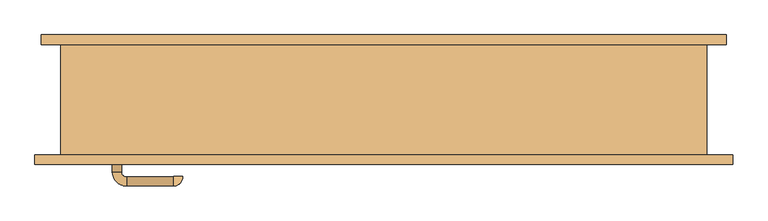
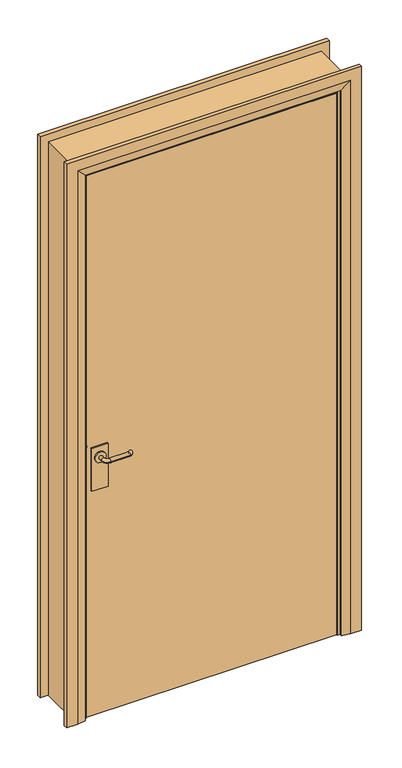
"""IFC4 building model written with IfcOpenShell, lengths in millimetres: door geometry, Porta Simples de Abrir : 90x210cm - Marco de Madeira."""

from ifc_helpers import new_model, si_unit, point, frame, frame_2d, origin, place, context, project, spatial, polyline, circle_curve, ellipse_curve, trimmed, segment, composite_curve, outline, extrude, faceted_brep, source, transform, mapped, element, save
from ifc_brep_helpers import plane_surface, cylinder_surface, revolved_surface, advanced_brep


def door_5ffc7892(model_context):
    return source(origin(), model_context, "Body", "SolidModel", [
        extrude(outline(composite_curve([segment(trimmed(circle_curve(frame_2d((1050.0, -413.0)), 20.0), [point((1050.0, -433.0))], [point((1050.0, -393.0))], False, "CARTESIAN"), True, "CONTINUOUS"), segment(trimmed(circle_curve(frame_2d((1050.0, -413.0)), 20.0), [point((1050.0, -393.0))], [point((1050.0, -433.0))], False, "CARTESIAN"), True, "CONTINUOUS")], self_intersect=False)), frame((0.0, -44.6, 0.0), z_axis=(0.0, 1.0, 0.0), x_axis=(0.0, 0.0, 1.0)), (0.0, 0.0, 1.0), 4.5929895),
        advanced_brep(
        [(-406.0, -40.0070105, 1050.0), (-420.0, -40.0070105, 1050.0), (-406.0, -24.6, 1050.0), (-420.0, -24.6, 1050.0), (-398.0, -2.6, 1050.0), (-398.0, -16.6, 1050.0), (-326.0, -16.6, 1050.0), (-326.0, -2.6, 1050.0), (-325.0, -17.6, 1050.0), (-311.0, -17.6, 1050.0)],
        [
            (0, 1, circle_curve(frame((-413.0, -40.0070105, 1050.0), z_axis=(0.0, -1.0, 0.0), x_axis=(-1.0, 0.0, 0.0)), 7.0)),
            (1, 0, circle_curve(frame((-413.0, -40.0070105, 1050.0), z_axis=(0.0, -1.0, 0.0), x_axis=(-1.0, 0.0, 0.0)), 7.0)),
            (0, 2),
            (2, 3, circle_curve(frame((-413.0, -24.6, 1050.0), z_axis=(0.0, -1.0, 0.0), x_axis=(-1.0, 0.0, 0.0)), 7.0)),
            (3, 1),
            (3, 2, circle_curve(frame((-413.0, -24.6, 1050.0), z_axis=(0.0, -1.0, 0.0), x_axis=(-1.0, 0.0, 0.0)), 7.0)),
            (4, 3, circle_curve(frame((-398.0, -24.6, 1050.0), z_axis=(0.0, 0.0, 1.0), x_axis=(-1.0, 0.0, 0.0)), 22.0)),
            (2, 5, circle_curve(frame((-398.0, -24.6, 1050.0), z_axis=(0.0, 0.0, -1.0), x_axis=(-1.0, 0.0, 0.0)), 8.0)),
            (5, 4, circle_curve(frame((-398.0, -9.6, 1050.0), z_axis=(-1.0, 0.0, 0.0), x_axis=(0.0, 1.0, 0.0)), 7.0)),
            (4, 5, circle_curve(frame((-398.0, -9.6, 1050.0), z_axis=(-1.0, 0.0, 0.0), x_axis=(0.0, 1.0, 0.0)), 7.0)),
            (5, 6),
            (6, 7, circle_curve(frame((-326.0, -9.6, 1050.0), z_axis=(-1.0, 0.0, 0.0), x_axis=(0.0, 1.0, 0.0)), 7.0)),
            (7, 4),
            (7, 6, circle_curve(frame((-326.0, -9.6, 1050.0), z_axis=(-1.0, 0.0, 0.0), x_axis=(0.0, 1.0, 0.0)), 7.0)),
            (8, 9, circle_curve(frame((-318.0, -17.6, 1050.0), z_axis=(0.0, -1.0, 0.0), x_axis=(1.0, 0.0, 0.0)), 7.0)),
            (9, 8, circle_curve(frame((-318.0, -17.6, 1050.0), z_axis=(0.0, -1.0, 0.0), x_axis=(1.0, 0.0, 0.0)), 7.0)),
            (9, 7, circle_curve(frame((-326.0, -17.6, 1050.0), z_axis=(0.0, 0.0, 1.0), x_axis=(0.0, 1.0, 0.0)), 15.0)),
            (6, 8, circle_curve(frame((-326.0, -17.6, 1050.0), z_axis=(0.0, 0.0, -1.0), x_axis=(0.0, 1.0, 0.0)), 1.0)),
        ],
        [
            plane_surface(frame((-413.0, -40.0070105, 1050.0), z_axis=(0.0, -1.0, 0.0), x_axis=(0.0, 0.0, 1.0))),
            cylinder_surface(frame((-413.0, -40.0070105, 1050.0), z_axis=(0.0, -1.0, 0.0), x_axis=(-1.0, 0.0, 0.0)), 7.0),
            revolved_surface(trimmed(ellipse_curve(frame((-413.0, -24.6, 1050.0), z_axis=(0.0, -1.0, 0.0), x_axis=(-1.0, 0.0, 0.0)), 7.0, 7.0), [point((-406.0, -24.6, 1050.0))], [point((-420.0, -24.6, 1050.0))], True, "CARTESIAN"), (-398.0, -24.6, 1050.0), (0.0, 0.0, -1.0)),
            revolved_surface(trimmed(ellipse_curve(frame((-413.0, -24.6, 1050.0), z_axis=(0.0, -1.0, 0.0), x_axis=(-1.0, 0.0, 0.0)), 7.0, 7.0), [point((-420.0, -24.6, 1050.0))], [point((-406.0, -24.6, 1050.0))], True, "CARTESIAN"), (-398.0, -24.6, 1050.0), (0.0, 0.0, -1.0)),
            cylinder_surface(frame((-398.0, -9.6, 1050.0), z_axis=(-1.0, 0.0, 0.0), x_axis=(0.0, 1.0, 0.0)), 7.0),
            plane_surface(frame((-318.0, -17.6, 1050.0), z_axis=(0.0, -1.0, 0.0), x_axis=(0.0, 0.0, 1.0))),
            revolved_surface(trimmed(ellipse_curve(frame((-326.0, -9.6, 1050.0), z_axis=(-1.0, 0.0, 0.0), x_axis=(0.0, 1.0, 0.0)), 7.0, 7.0), [point((-326.0, -16.6, 1050.0))], [point((-326.0, -2.6, 1050.0))], True, "CARTESIAN"), (-326.0, -17.6, 1050.0), (0.0, 0.0, -1.0)),
            revolved_surface(trimmed(ellipse_curve(frame((-326.0, -9.6, 1050.0), z_axis=(-1.0, 0.0, 0.0), x_axis=(0.0, 1.0, 0.0)), 7.0, 7.0), [point((-326.0, -2.6, 1050.0))], [point((-326.0, -16.6, 1050.0))], True, "CARTESIAN"), (-326.0, -17.6, 1050.0), (0.0, 0.0, -1.0)),
        ],
        [
            (0, [[1, 2]]),
            (1, [[-1, 3, 4, 5]]),
            (1, [[-2, -5, 6, -3]]),
            (2, [[7, -4, 8, 9]]),
            (3, [[-8, -6, -7, 10]]),
            (4, [[-9, 11, 12, 13]]),
            (4, [[-10, -13, 14, -11]]),
            (5, [[15, 16]]),
            (6, [[17, -12, 18, -16]]),
            (7, [[-18, -14, -17, -15]]),
        ],
    ),
        extrude(outline(polyline([(-383.0, -50.6), (-443.0, -50.6), (-443.0, -44.6), (-383.0, -44.6), (-383.0, -50.6)])), frame((0.0, 0.0, 925.0), z_axis=(0.0, 0.0, 1.0), x_axis=(1.0, 0.0, 0.0)), (0.0, 0.0, 1.0), 165.0),
        extrude(outline(composite_curve([segment(trimmed(circle_curve(frame_2d((1050.0, -413.0)), 20.0), [point((1050.0, -433.0))], [point((1050.0, -393.0))], False, "CARTESIAN"), True, "CONTINUOUS"), segment(trimmed(circle_curve(frame_2d((1050.0, -413.0)), 20.0), [point((1050.0, -393.0))], [point((1050.0, -433.0))], False, "CARTESIAN"), True, "CONTINUOUS")], self_intersect=False)), frame((0.0, -96.1929895, 0.0), z_axis=(0.0, 1.0, 0.0), x_axis=(0.0, 0.0, 1.0)), (0.0, 0.0, 1.0), 4.5929895),
        advanced_brep(
        [(-406.0, -96.1929895, 1050.0), (-420.0, -96.1929895, 1050.0), (-420.0, -111.6, 1050.0), (-406.0, -111.6, 1050.0), (-398.0, -133.6, 1050.0), (-398.0, -119.6, 1050.0), (-326.0, -133.6, 1050.0), (-326.0, -119.6, 1050.0), (-325.0, -118.6, 1050.0), (-311.0, -118.6, 1050.0)],
        [
            (0, 1, circle_curve(frame((-413.0, -96.1929895, 1050.0), z_axis=(0.0, 1.0, 0.0), x_axis=(-1.0, 0.0, 0.0)), 7.0)),
            (1, 0, circle_curve(frame((-413.0, -96.1929895, 1050.0), z_axis=(0.0, 1.0, 0.0), x_axis=(-1.0, 0.0, 0.0)), 7.0)),
            (1, 2),
            (2, 3, circle_curve(frame((-413.0, -111.6, 1050.0), z_axis=(0.0, 1.0, 0.0), x_axis=(-1.0, 0.0, 0.0)), 7.0)),
            (3, 0),
            (3, 2, circle_curve(frame((-413.0, -111.6, 1050.0), z_axis=(0.0, 1.0, 0.0), x_axis=(-1.0, 0.0, 0.0)), 7.0)),
            (4, 5, circle_curve(frame((-398.0, -126.6, 1050.0), z_axis=(-1.0, 0.0, 0.0), x_axis=(0.0, -1.0, 0.0)), 7.0)),
            (5, 3, circle_curve(frame((-398.0, -111.6, 1050.0), z_axis=(0.0, 0.0, -1.0), x_axis=(-1.0, 0.0, 0.0)), 8.0)),
            (2, 4, circle_curve(frame((-398.0, -111.6, 1050.0), z_axis=(0.0, 0.0, 1.0), x_axis=(-1.0, 0.0, 0.0)), 22.0)),
            (5, 4, circle_curve(frame((-398.0, -126.6, 1050.0), z_axis=(-1.0, 0.0, 0.0), x_axis=(0.0, -1.0, 0.0)), 7.0)),
            (4, 6),
            (6, 7, circle_curve(frame((-326.0, -126.6, 1050.0), z_axis=(-1.0, 0.0, 0.0), x_axis=(0.0, -1.0, 0.0)), 7.0)),
            (7, 5),
            (7, 6, circle_curve(frame((-326.0, -126.6, 1050.0), z_axis=(-1.0, 0.0, 0.0), x_axis=(0.0, -1.0, 0.0)), 7.0)),
            (8, 9, circle_curve(frame((-318.0, -118.6, 1050.0), z_axis=(0.0, 1.0, 0.0), x_axis=(1.0, 0.0, 0.0)), 7.0)),
            (9, 8, circle_curve(frame((-318.0, -118.6, 1050.0), z_axis=(0.0, 1.0, 0.0), x_axis=(1.0, 0.0, 0.0)), 7.0)),
            (8, 7, circle_curve(frame((-326.0, -118.6, 1050.0), z_axis=(0.0, 0.0, -1.0), x_axis=(0.0, -1.0, 0.0)), 1.0)),
            (6, 9, circle_curve(frame((-326.0, -118.6, 1050.0), z_axis=(0.0, 0.0, 1.0), x_axis=(0.0, -1.0, 0.0)), 15.0)),
        ],
        [
            plane_surface(frame((-413.0, -96.1929895, 1050.0), z_axis=(0.0, 1.0, 0.0), x_axis=(0.0, 0.0, 1.0))),
            cylinder_surface(frame((-413.0, -96.1929895, 1050.0), z_axis=(0.0, 1.0, 0.0), x_axis=(-1.0, 0.0, 0.0)), 7.0),
            revolved_surface(trimmed(ellipse_curve(frame((-413.0, -111.6, 1050.0), z_axis=(0.0, -1.0, 0.0), x_axis=(-1.0, 0.0, 0.0)), 7.0, 7.0), [point((-406.0, -111.6, 1050.0))], [point((-420.0, -111.6, 1050.0))], True, "CARTESIAN"), (-398.0, -111.6, 1050.0), (0.0, 0.0, -1.0)),
            revolved_surface(trimmed(ellipse_curve(frame((-413.0, -111.6, 1050.0), z_axis=(0.0, -1.0, 0.0), x_axis=(-1.0, 0.0, 0.0)), 7.0, 7.0), [point((-420.0, -111.6, 1050.0))], [point((-406.0, -111.6, 1050.0))], True, "CARTESIAN"), (-398.0, -111.6, 1050.0), (0.0, 0.0, -1.0)),
            cylinder_surface(frame((-398.0, -126.6, 1050.0), z_axis=(-1.0, 0.0, 0.0), x_axis=(0.0, -1.0, 0.0)), 7.0),
            plane_surface(frame((-318.0, -118.6, 1050.0), z_axis=(0.0, 1.0, 0.0), x_axis=(0.0, 0.0, 1.0))),
            revolved_surface(trimmed(ellipse_curve(frame((-326.0, -126.6, 1050.0), z_axis=(1.0, 0.0, 0.0), x_axis=(0.0, -1.0, 0.0)), 7.0, 7.0), [point((-326.0, -119.6, 1050.0))], [point((-326.0, -133.6, 1050.0))], True, "CARTESIAN"), (-326.0, -118.6, 1050.0), (0.0, 0.0, -1.0)),
            revolved_surface(trimmed(ellipse_curve(frame((-326.0, -126.6, 1050.0), z_axis=(1.0, 0.0, 0.0), x_axis=(0.0, -1.0, 0.0)), 7.0, 7.0), [point((-326.0, -133.6, 1050.0))], [point((-326.0, -119.6, 1050.0))], True, "CARTESIAN"), (-326.0, -118.6, 1050.0), (0.0, 0.0, -1.0)),
        ],
        [
            (0, [[1, 2]]),
            (1, [[3, 4, 5, -2]]),
            (1, [[-5, 6, -3, -1]]),
            (2, [[7, 8, -4, 9]]),
            (3, [[10, -9, -6, -8]]),
            (4, [[11, 12, 13, -7]]),
            (4, [[-13, 14, -11, -10]]),
            (5, [[15, 16]]),
            (6, [[-15, 17, -12, 18]]),
            (7, [[-16, -18, -14, -17]]),
        ],
    ),
        extrude(outline(polyline([(-383.0, -85.6), (-383.0, -91.6), (-443.0, -91.6), (-443.0, -85.6), (-383.0, -85.6)])), frame((0.0, 0.0, 925.0), z_axis=(0.0, 0.0, 1.0), x_axis=(1.0, 0.0, 0.0)), (0.0, 0.0, 1.0), 165.0),
        extrude(outline(polyline([(457.0, -50.6), (457.0, -85.6), (-457.0, -85.6), (-457.0, -50.6), (457.0, -50.6)])), frame((0.0, 0.0, 53.0), z_axis=(0.0, 0.0, 1.0), x_axis=(1.0, 0.0, 0.0)), (0.0, 0.0, 1.0), 2094.0),
        faceted_brep([(530.0, 85.6, 50.0), (460.0, 85.6, 50.0), (460.0, 95.6, 50.0), (490.0, 100.6, 50.0), (530.0, 100.6, 50.0), (530.0, 100.6, 2220.0), (530.0, 85.6, 2220.0), (490.0, 100.6, 2180.0), (-490.0, 100.6, 2180.0), (-490.0, 100.6, 50.0), (-530.0, 100.6, 50.0), (-530.0, 100.6, 2220.0), (460.0, 95.6, 2150.0), (460.0, 85.6, 2150.0), (-530.0, 85.6, 2220.0), (-530.0, 85.6, 50.0), (-460.0, 85.6, 50.0), (-460.0, 85.6, 2150.0), (-460.0, 95.6, 50.0), (-460.0, 95.6, 2150.0)], [[[0, 1, 2, 3, 4]], [[4, 5, 6, 0]], [[3, 7, 8, 9, 10, 11, 5, 4]], [[2, 12, 7, 3]], [[1, 13, 12, 2]], [[0, 6, 14, 15, 16, 17, 13, 1]], [[17, 16, 18, 19]], [[15, 10, 9, 18, 16]], [[11, 10, 15, 14]], [[19, 18, 9, 8]], [[13, 17, 19, 12]], [[5, 11, 14, 6]], [[12, 19, 8, 7]]]),
        faceted_brep([(540.0, -85.6, 50.0), (540.0, -100.6, 50.0), (500.0, -100.6, 50.0), (470.0, -95.6, 50.0), (470.0, -85.6, 50.0), (470.0, -85.6, 2160.0), (-470.0, -85.6, 2160.0), (-470.0, -85.6, 50.0), (-540.0, -85.6, 50.0), (-540.0, -85.6, 2230.0), (540.0, -85.6, 2230.0), (470.0, -95.6, 2160.0), (500.0, -100.6, 2190.0), (540.0, -100.6, 2230.0), (-540.0, -100.6, 2230.0), (-540.0, -100.6, 50.0), (-500.0, -100.6, 50.0), (-500.0, -100.6, 2190.0), (-470.0, -95.6, 50.0), (-470.0, -95.6, 2160.0)], [[[0, 1, 2, 3, 4]], [[4, 5, 6, 7, 8, 9, 10, 0]], [[3, 11, 5, 4]], [[2, 12, 11, 3]], [[1, 13, 14, 15, 16, 17, 12, 2]], [[0, 10, 13, 1]], [[9, 8, 15, 14]], [[8, 7, 18, 16, 15]], [[19, 18, 7, 6]], [[17, 16, 18, 19]], [[11, 19, 6, 5]], [[10, 9, 14, 13]], [[12, 17, 19, 11]]]),
        faceted_brep([(-460.0, -85.6, 50.0), (-500.0, -85.6, 50.0), (-500.0, 85.6, 50.0), (-450.0, 85.6, 50.0), (-450.0, -47.6, 50.0), (-460.0, -47.6, 50.0), (-460.0, -85.6, 2150.0), (-500.0, -85.6, 2190.0), (-500.0, 85.6, 2190.0), (-450.0, 85.6, 2140.0), (-450.0, -47.6, 2140.0), (-460.0, -47.6, 2150.0), (460.0, -85.6, 50.0), (460.0, -47.6, 50.0), (450.0, -47.6, 50.0), (450.0, 85.6, 50.0), (500.0, 85.6, 50.0), (500.0, -85.6, 50.0), (460.0, -47.6, 2150.0), (460.0, -85.6, 2150.0), (450.0, -47.6, 2140.0), (450.0, 85.6, 2140.0), (500.0, 85.6, 2190.0), (500.0, -85.6, 2190.0)], [[[0, 1, 2, 3, 4, 5]], [[0, 6, 7, 1]], [[1, 7, 8, 2]], [[2, 8, 9, 3]], [[3, 9, 10, 4]], [[4, 10, 11, 5]], [[5, 11, 6, 0]], [[12, 13, 14, 15, 16, 17]], [[18, 13, 12, 19]], [[20, 14, 13, 18]], [[21, 15, 14, 20]], [[22, 16, 15, 21]], [[23, 17, 16, 22]], [[19, 12, 17, 23]], [[6, 19, 23, 7]], [[7, 23, 22, 8]], [[8, 22, 21, 9]], [[9, 21, 20, 10]], [[10, 20, 18, 11]], [[11, 18, 19, 6]]]),
    ])


if __name__ == "__main__":
    model = new_model("IFC4")
    model_context = context("Model", 3, world=origin())
    ifc_project = project(units=[si_unit("LENGTHUNIT", "METRE", prefix="MILLI")], contexts=[model_context])
    site = spatial("IfcSite", under=ifc_project)
    building = spatial("IfcBuilding", under=site)
    placement = place(None, origin())
    door_shape = door_5ffc7892(model_context)
    element("IfcDoor", 1, ObjectType="Porta Simples de Abrir : 90x210cm - Marco de Madeira", at=placement, inside=building, context=model_context, shape_type="MappedRepresentation", body=[
        mapped(door_shape, transform((0.0, 0.0, 0.0), x_axis=(1.0, 0.0, 0.0), y_axis=(0.0, 1.0, 0.0), z_axis=(0.0, 0.0, 1.0))),
    ])
    save(model, "model.ifc")

# Revit data of these elements
# Type "Porta Simples de Abrir : 90x210cm - Marco de Madeira"
#   Type Mark = ""
#   SINAPI = ""
#   Construction Type = "300"
#   Maçaneta [instance default] = ""
#   Fechadura [instance default] = ""
#   Vão Luz (somente para informação) = 88.00 cm
#   Tolerância Folha Vertical = 0.30 cm
#   Módulo Básico M = 10.00 cm
#   Largura de Coordenação Modular Largura CM = 100.00 cm
#   Rough Width = 100.00 cm
#   Deslocamento da Horizontal da Folha = 0.00 cm
#   Altura de Coordenação Modular Largura CM = 220.00 cm
#   Rough Height = 220.00 cm
#   Altura Nominal = 209.00 cm
#   Ajuste de Coordenação Topo AC Topo = 1.00 cm
#   Ajuste de Coordenação Base AC Base = 5.00 cm
#   Ajuste de Coordenação AC = 1.00 cm
#   Tolerância Folha Horizontal = 0.30 cm
#   Largura Folha (somente para informação) = 89.40 cm
#   Espessura Folha = 3.50 cm
#   Maçaneta - Distância da Folha = 4.40 cm
#   Maçaneta - Altura = 100.00 cm
#   Largura Nominal (Largura Mn) = 92.00 cm
#   Distância do Nível = 0.30 cm
#   Aduela Interna Espessura = 4.00 cm
#   Aduela Externa Espessura = 5.00 cm
#   Altura Folha (somente para informação) = 207.40 cm
#   Height = 214.00 cm
#   Width = 98.00 cm
#   Número de Módulos Básicos nM Largura = 10
#   Número de Módulos Básicos nM Altura = 22
#   Marco Metálico = no
#   Aduela de Madeira = no
#   Aduela Metálica de Canto = no
#   Guarnição Reta = no
#   Guarnição Chanfrada = yes
#   Batente - Material [instance default] = none
#   Painel - Material [instance default] = none
#   Model = ""
#   Function = (empty or 0)
#   Description = (empty or 0)
#   Wall Closure = (empty or 0)
#   Assembly Code = ""
# Element 1 (IfcDoor, "Porta Simples de Abrir : 90x210cm - Marco de Madeira")
#   Materials on its faces: "Porta - Maçaneta"
# Materials
#   "Porta - Maçaneta": class "Metal", colour RGB 189 187 185, transparency 0, Cost = 0
